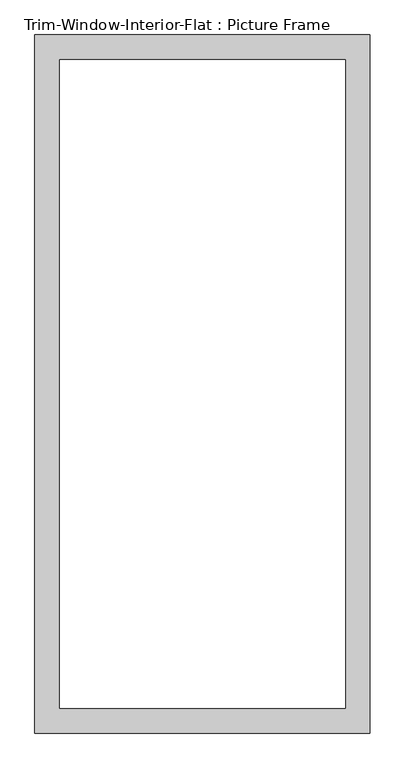
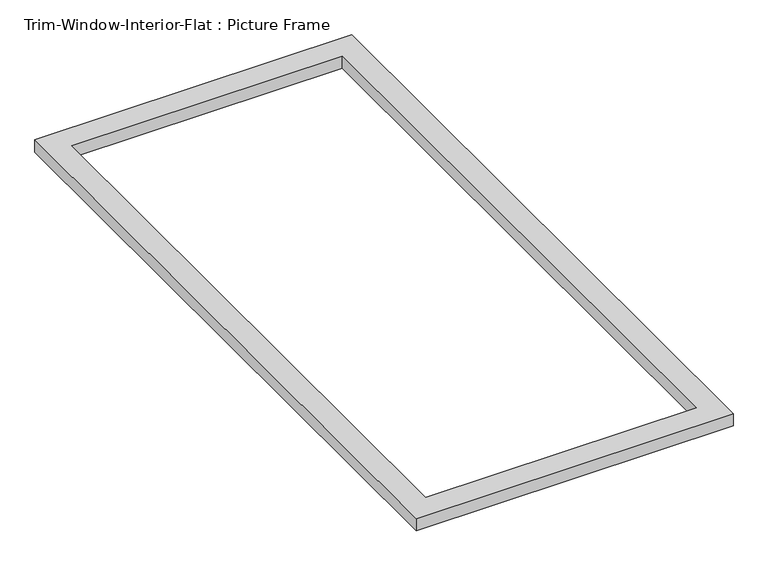
"""IFC4 building model written with IfcOpenShell, lengths in millimetres: proxy geometry, Trim-Window-Interior-Flat : Picture Frame."""

from ifc_helpers import new_model, si_unit, origin, origin_with_axes, place, context, project, spatial, polyline, outline, extrude, source, transform, mapped, element, save


def trim_window_interior_flat_picture_frame_3fc80fe0(model_context):
    return source(origin(), model_context, "Body", "SweptSolid", [
        extrude(outline(polyline([(387.35, 44.45), (387.35, -1568.45), (-387.35, -1568.45), (-387.35, 44.45), (387.35, 44.45)]), holes=[polyline([(330.2, -12.7), (-330.2, -12.7), (-330.2, -1511.3), (330.2, -1511.3), (330.2, -12.7)])]), origin_with_axes(), (0.0, 0.0, 1.0), 31.75),
    ])


if __name__ == "__main__":
    model = new_model("IFC4")
    model_context = context("Model", 3, world=origin())
    ifc_project = project(units=[si_unit("LENGTHUNIT", "METRE", prefix="MILLI")], contexts=[model_context])
    site = spatial("IfcSite", under=ifc_project)
    building = spatial("IfcBuilding", under=site)
    placement = place(None, origin())
    trim_window_interior_flat_picture_frame_shape = trim_window_interior_flat_picture_frame_3fc80fe0(model_context)
    element("IfcBuildingElementProxy", 1, Name="Trim-Window-Interior-Flat : Picture Frame", ObjectType="Trim-Window-Interior-Flat : Picture Frame", at=placement, inside=building, context=model_context, shape_type="MappedRepresentation", body=[
        mapped(trim_window_interior_flat_picture_frame_shape, transform((0.0, 0.0, 0.0), x_axis=(1.0, 0.0, 0.0), y_axis=(0.0, 1.0, 0.0), z_axis=(0.0, 0.0, 1.0))),
    ])
    save(model, "model.ifc")

# Revit data of these elements
# Type "Trim-Window-Interior-Flat : Picture Frame"
#   Trim Thickness_Picture Frame = 0' - 1 1/4"
#   Trim Width = 0' - 2 1/4"
#   Trim Thickness_with Sill = 0' - 0 3/4"
#   Sill Thickness = 0' - 1 1/4"
#   Opening Width [instance default] = 2' - 0"
#   Opening Height [instance default] = 3' - 0"
#   Default Elevation = 4' - 0"
#   Sill = no
#   Picture Frame = yes
#   Trim Material [instance default] = none
# Element 1 (IfcBuildingElementProxy, "Trim-Window-Interior-Flat : Picture Frame")
#   Opening Width = 2' - 3"
#   Opening Height = 5' - 0"
#   Trim Material = Wood - Stained
#   Materials on its faces: "Wood - Stained"
# Materials
#   "Wood - Stained": class "Wood", colour RGB 224 178 126, transparency 0, Cost = 0
